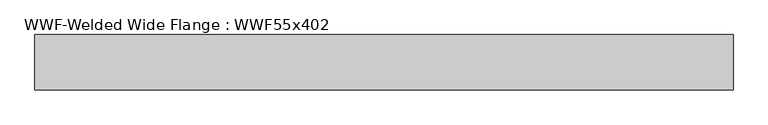
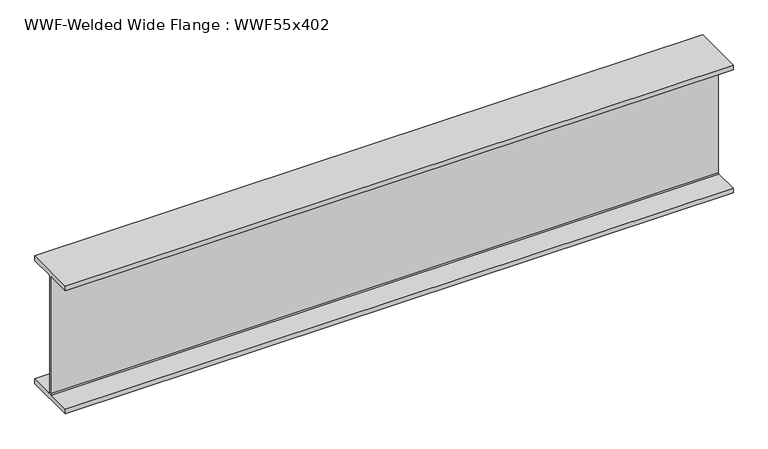
"""IFC4 building model written with IfcOpenShell, lengths in millimetres: beam geometry, WWF-Welded Wide Flange : WWF55x402."""

from ifc_helpers import new_model, si_unit, frame, origin, place, context, project, spatial, polyline, outline, extrude, source, transform, mapped, element, save


def wwf_welded_wide_flange_wwf55x402_d8a73b6f(model_context):
    return source(origin(), model_context, "Body", "SweptSolid", [
        extrude(outline(polyline([(274.955, -649.986), (274.955, -700.024), (-274.955, -700.024), (-274.955, -649.986), (-19.05, -649.986), (-8.001, -638.937), (-8.001, 638.937), (-19.05, 649.986), (-274.955, 649.986), (-274.955, 700.024), (274.955, 700.024), (274.955, 649.986), (19.05, 649.986), (8.001, 638.937), (8.001, -638.937), (19.05, -649.986), (274.955, -649.986)])), frame((-3472.2200653, 0.0, 0.0), z_axis=(1.0, 0.0, 0.0), x_axis=(0.0, 1.0, 0.0)), (0.0, 0.0, 1.0), 6931.74013),
    ])


if __name__ == "__main__":
    model = new_model("IFC4")
    model_context = context("Model", 3, world=origin())
    ifc_project = project(units=[si_unit("LENGTHUNIT", "METRE", prefix="MILLI")], contexts=[model_context])
    site = spatial("IfcSite", under=ifc_project)
    building = spatial("IfcBuilding", under=site)
    placement = place(None, origin())
    wwf_welded_wide_flange_wwf55x402_shape = wwf_welded_wide_flange_wwf55x402_d8a73b6f(model_context)
    element("IfcBeam", 1, ObjectType="WWF-Welded Wide Flange : WWF55x402", at=placement, inside=building, context=model_context, shape_type="MappedRepresentation", body=[
        mapped(wwf_welded_wide_flange_wwf55x402_shape, transform((0.0, 0.0, 0.0), x_axis=(1.0, 0.0, 0.0), y_axis=(0.0, 1.0, 0.0), z_axis=(0.0, 0.0, 1.0))),
    ])
    save(model, "model.ifc")

# Revit data of these elements
# Type "WWF-Welded Wide Flange : WWF55x402"
#   Assembly Code = "B10"
#   Nominal d = "12"
#   W = 402
#   Length [instance default] = 1524 mm
#   bf = 549.91 mm
#   d = 1400.048 mm
#   k = 19.05 mm
#   tf = 50.038 mm
#   tw = 16.002 mm
#   A = 0.0761289 m²
#   Structural Material [instance default] = Steel ASTM A572
# Element 1 (IfcBeam, "WWF-Welded Wide Flange : WWF55x402")
#   Structural Material = Metal - Steel 43-275
#   Materials on its faces: "Metal - Steel 43-275"
# Materials
#   "Steel ASTM A572": class "Metal", colour RGB 247 247 247, transparency 0, Description = "Structural steel, high strength low alloy, ASTM - A572 - 50", Cost = 0
#   "Metal - Steel 43-275": class "Metal", colour RGB 247 247 247, transparency 0, Cost = 0
